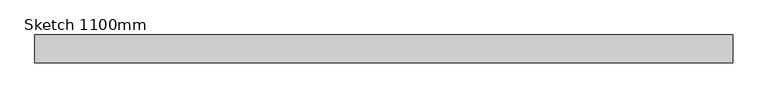
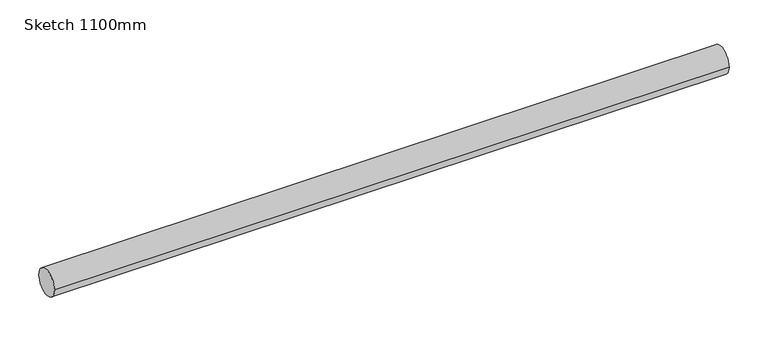
"""IFC4 building model written with IfcOpenShell, lengths in millimetres: railing geometry, Sketch 1100mm."""

import ifcopenshell
import ifcopenshell.guid

model = None  # the IFC model being written
_history = None  # IfcOwnerHistory: only IFC2X3 demands one
_inside = {}  # id of a spatial element -> (the spatial element, [elements in it])
_under = {}  # id of a project, library or spatial element -> (it, [spatial elements below it])
_declared = {}  # id of a project -> (the project, [libraries it declares])
_typed = {}  # id of a type object -> (the type object, [elements of that type])
_made_of = {}  # id of a material, layer set ... -> (it, [elements and type objects made of it])


def new_model(schema):
    """Start an empty IFC model of exactly this schema.

    Asked for "IFC4X3", IfcOpenShell would pick the latest addendum, in which some entities
    have other attributes; the version numbers below select the first issue.
    IFC2X3 requires an IfcOwnerHistory on every rooted entity: one is made here for all.
    """
    global model, _history
    if schema == "IFC4X3":
        model = ifcopenshell.file(schema_version=(4, 3, 0, 0))
    else:
        model = ifcopenshell.file(schema=schema)
    _inside.clear()
    _under.clear()
    _declared.clear()
    _typed.clear()
    _made_of.clear()
    _history = None
    if model.schema == "IFC2X3":
        org = make("IfcOrganization", Name="unknown")
        user = make(
            "IfcPersonAndOrganization",
            ThePerson=make("IfcPerson", FamilyName="unknown"),
            TheOrganization=org,
        )
        app = make(
            "IfcApplication",
            ApplicationDeveloper=org,
            Version="unknown",
            ApplicationFullName="unknown",
            ApplicationIdentifier="unknown",
        )
        _history = make(
            "IfcOwnerHistory",
            OwningUser=user,
            OwningApplication=app,
            ChangeAction="ADDED",
            CreationDate=0,
        )
    return model


def make(cls, **values):
    """One entity of the class cls with the attributes given. An attribute that is None is left unset."""
    return model.create_entity(
        cls, **{name: value for name, value in values.items() if value is not None}
    )


def rooted(cls, **values):
    """An entity with a GlobalId (a new one), such as an element, a storey or a relation."""
    return make(cls, GlobalId=ifcopenshell.guid.new(), OwnerHistory=_history, **values)


def si_unit(unit_type, name, prefix=None):
    """IfcSIUnit, for example si_unit("LENGTHUNIT", "METRE", prefix="MILLI")."""
    return make("IfcSIUnit", UnitType=unit_type, Prefix=prefix, Name=name)


def assignment(units):
    """IfcUnitAssignment: the units of a project."""
    return None if units is None else make("IfcUnitAssignment", Units=units)


def point(xyz):
    """IfcCartesianPoint."""
    return None if xyz is None else make("IfcCartesianPoint", Coordinates=xyz)


def direction(xyz):
    """IfcDirection."""
    return None if xyz is None else make("IfcDirection", DirectionRatios=xyz)


def frame(location, z_axis=None, x_axis=None):
    """IfcAxis2Placement3D, a coordinate frame: its origin and axes. An axis left out is left unset."""
    return make(
        "IfcAxis2Placement3D",
        Location=point(location),
        Axis=direction(z_axis),
        RefDirection=direction(x_axis),
    )


def frame_2d(location, x_axis=None):
    """IfcAxis2Placement2D, a coordinate frame in the plane: its origin and x axis."""
    return make(
        "IfcAxis2Placement2D", Location=point(location), RefDirection=direction(x_axis)
    )


def origin():
    """The frame at (0, 0, 0) with its axes left unset."""
    return frame((0.0, 0.0, 0.0))


def place(relative_to, where):
    """IfcLocalPlacement: puts the frame where relative to a parent placement (None: the world)."""
    return make(
        "IfcLocalPlacement", PlacementRelTo=relative_to, RelativePlacement=where
    )


def context(
    kind, dimensions, precision=None, world=None, true_north=None, identifier=None
):
    """IfcGeometricRepresentationContext, for example the 3D "Model" context."""
    return make(
        "IfcGeometricRepresentationContext",
        ContextIdentifier=identifier,
        ContextType=kind,
        CoordinateSpaceDimension=dimensions,
        Precision=precision,
        WorldCoordinateSystem=world,
        TrueNorth=true_north,
    )


def project(units=None, contexts=None):
    """IfcProject with its units and contexts."""
    return rooted(
        "IfcProject",
        Name="project",
        RepresentationContexts=contexts,
        UnitsInContext=assignment(units),
    )


def spatial(cls, under=None, at=None, **own):
    """A site, building, storey or space (cls), placed at a placement, below another one or the project."""
    s = rooted(cls, ObjectPlacement=at, **own)
    if under is not None:
        _under.setdefault(under.id(), (under, []))[1].append(s)
    return s


def circle_curve(where, radius):
    """IfcCircle in the frame where."""
    return make("IfcCircle", Position=where, Radius=radius)


def trimmed(basis, trim1, trim2, sense, master):
    """IfcTrimmedCurve: the piece of a basis curve between two trims."""
    return make(
        "IfcTrimmedCurve",
        BasisCurve=basis,
        Trim1=trim1,
        Trim2=trim2,
        SenseAgreement=sense,
        MasterRepresentation=master,
    )


def segment(curve, same_sense, transition):
    """IfcCompositeCurveSegment."""
    return make(
        "IfcCompositeCurveSegment",
        Transition=transition,
        SameSense=same_sense,
        ParentCurve=curve,
    )


def composite_curve(segments, self_intersect=None):
    """IfcCompositeCurve: segments joined end to end."""
    return make("IfcCompositeCurve", Segments=segments, SelfIntersect=self_intersect)


def outline(outer, holes=None, kind="AREA"):
    """IfcArbitraryClosedProfileDef: a profile drawn as a closed curve; with holes, ...WithVoids."""
    if holes is None:
        return make("IfcArbitraryClosedProfileDef", ProfileType=kind, OuterCurve=outer)
    return make(
        "IfcArbitraryProfileDefWithVoids",
        ProfileType=kind,
        OuterCurve=outer,
        InnerCurves=holes,
    )


def extrude(swept, where, along, depth):
    """IfcExtrudedAreaSolid: the profile swept, set in the frame where, extruded along a direction by depth."""
    return make(
        "IfcExtrudedAreaSolid",
        SweptArea=swept,
        Position=where,
        ExtrudedDirection=direction(along),
        Depth=depth,
    )


def shape(context_of_items, identifier, shape_type, items):
    """IfcShapeRepresentation: the items that make up one representation, for example the "Body"."""
    return make(
        "IfcShapeRepresentation",
        ContextOfItems=context_of_items,
        RepresentationIdentifier=identifier,
        RepresentationType=shape_type,
        Items=items,
    )


def source(mapping_origin, context_of_items, identifier, shape_type, items):
    """IfcRepresentationMap: a shape defined once, which mapped items show again and again."""
    return make(
        "IfcRepresentationMap",
        MappingOrigin=mapping_origin,
        MappedRepresentation=shape(context_of_items, identifier, shape_type, items),
    )


def transform(
    local_origin,
    x_axis=None,
    y_axis=None,
    z_axis=None,
    scale=None,
    scale2=None,
    scale3=None,
    uniform=True,
):
    """IfcCartesianTransformationOperator3D, or its non-uniform kind. x_axis, y_axis, z_axis: its Axis1, 2, 3."""
    if uniform:
        return make(
            "IfcCartesianTransformationOperator3D",
            Axis1=direction(x_axis),
            Axis2=direction(y_axis),
            LocalOrigin=point(local_origin),
            Scale=scale,
            Axis3=direction(z_axis),
        )
    return make(
        "IfcCartesianTransformationOperator3DnonUniform",
        Axis1=direction(x_axis),
        Axis2=direction(y_axis),
        LocalOrigin=point(local_origin),
        Scale=scale,
        Axis3=direction(z_axis),
        Scale2=scale2,
        Scale3=scale3,
    )


def mapped(mapping_source, mapping_target):
    """IfcMappedItem: shows the shape of a source again, moved by a transform."""
    return make(
        "IfcMappedItem", MappingSource=mapping_source, MappingTarget=mapping_target
    )


def made_of(thing, what):
    """Note that an element or type object is made of a material, layer set ...; save() writes the relation."""
    if what is not None:
        _made_of.setdefault(what.id(), (what, []))[1].append(thing)
    return thing


def element(
    cls,
    number,
    at=None,
    inside=None,
    cuts=None,
    type_object=None,
    material=None,
    context=None,
    identifier="Body",
    shape_type=None,
    held_by="IfcProductDefinitionShape",
    body=None,
    shapes=None,
    **own,
):
    """One element of the class cls, such as IfcWall. Its Tag is "e" and its number.

    at: its placement. inside: the storey or other place that contains it. cuts: it is an
    opening in that element (IfcRelVoidsElement). A single representation is given by context,
    identifier, shape_type and body (its items); several are given by shapes. held_by: the class
    of the entity that holds the representations. save() writes the other relations.
    """
    e = rooted(cls, Tag="e%d" % number, ObjectPlacement=at, **own)
    if body is not None:
        shapes = [shape(context, identifier, shape_type, body)]
    if shapes is not None:
        e.Representation = make(held_by, Representations=shapes)
    if inside is not None:
        _inside.setdefault(inside.id(), (inside, []))[1].append(e)
    if cuts is not None:
        rooted(
            "IfcRelVoidsElement", RelatingBuildingElement=cuts, RelatedOpeningElement=e
        )
    if type_object is not None:
        _typed.setdefault(type_object.id(), (type_object, []))[1].append(e)
    return made_of(e, material)


def aggregate(whole, parts):
    """IfcRelAggregates: a whole, such as a stair, and the parts it consists of."""
    return rooted("IfcRelAggregates", RelatingObject=whole, RelatedObjects=parts)


def save(model, path):
    """Write the relations noted so far, then the file.

    IfcRelAggregates (storeys below a building ...), IfcRelContainedInSpatialStructure (elements
    in a storey), IfcRelDefinesByType, IfcRelAssociatesMaterial and IfcRelDeclares: one each for
    every whole, place, type object, material and project.
    """
    for whole, parts in _under.values():
        aggregate(whole, parts)
    for where, things in _inside.values():
        rooted(
            "IfcRelContainedInSpatialStructure",
            RelatedElements=things,
            RelatingStructure=where,
        )
    for kind, things in _typed.values():
        rooted("IfcRelDefinesByType", RelatedObjects=things, RelatingType=kind)
    for what, things in _made_of.values():
        rooted("IfcRelAssociatesMaterial", RelatedObjects=things, RelatingMaterial=what)
    for by, libraries in _declared.values():
        rooted("IfcRelDeclares", RelatingContext=by, RelatedDefinitions=libraries)
    model.write(path)


def sketch_1100mm_82aaa055(model_context):
    return source(origin(), model_context, "Body", "SweptSolid", [
        extrude(outline(composite_curve([segment(trimmed(circle_curve(frame_2d((5300.0, 7480.0)), 20.0), [point((5280.0, 7480.0))], [point((5320.0, 7480.0))], False, "CARTESIAN"), True, "CONTINUOUS"), segment(trimmed(circle_curve(frame_2d((5300.0, 7480.0)), 20.0), [point((5320.0, 7480.0))], [point((5280.0, 7480.0))], False, "CARTESIAN"), True, "CONTINUOUS")], self_intersect=False)), frame((7925.0, 0.0, 0.0), z_axis=(1.0, 0.0, 0.0), x_axis=(0.0, 1.0, 0.0)), (0.0, 0.0, 1.0), 1000.0),
    ])


if __name__ == "__main__":
    model = new_model("IFC4")
    model_context = context("Model", 3, world=origin())
    ifc_project = project(units=[si_unit("LENGTHUNIT", "METRE", prefix="MILLI")], contexts=[model_context])
    site = spatial("IfcSite", under=ifc_project)
    building = spatial("IfcBuilding", under=site)
    placement = place(None, origin())
    sketch_1100mm_shape = sketch_1100mm_82aaa055(model_context)
    element("IfcRailing", 1, ObjectType="Sketch 1100mm", at=placement, inside=building, context=model_context, shape_type="MappedRepresentation", body=[
        mapped(sketch_1100mm_shape, transform((0.0, 0.0, 0.0), x_axis=(1.0, 0.0, 0.0), y_axis=(0.0, 1.0, 0.0), z_axis=(0.0, 0.0, 1.0))),
    ])
    save(model, "model.ifc")

# Revit data of these elements
# Project information
#   Template Version = "DanEDU Building template ver. 2018.0420.0"
#   Client Name = "Test Project"
#   Project Address = "Enter address here"
#   Project Name = "3 Stories"
#   Project Number = "Number"
#   Current Version = "0.0.0"
#   SR Document GUID = "3eb9317e-835d-4f79-8926-4d15b96bc824"
# Element 1 (IfcRailing, "Sketch 1100mm")
#   Materials on its faces: "Default Railings (Interior/Exterior)"
# Materials
#   "Default Railings (Interior/Exterior)": class "Generic", colour RGB 205 205 205, transparency 0, Description = "Udefineret gelænder materiale", Cost = 0
